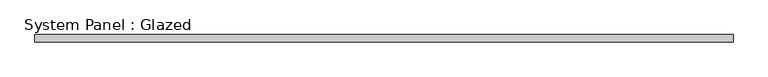
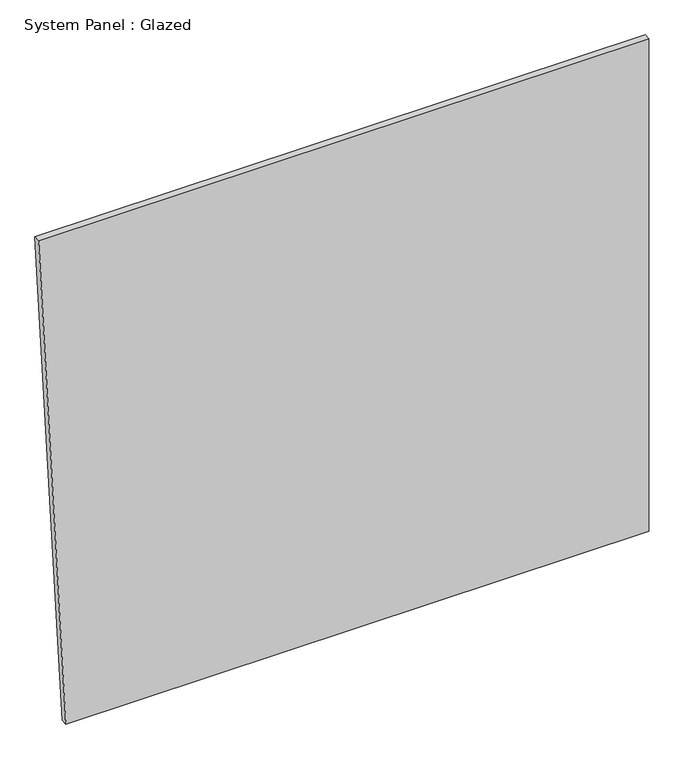
"""IFC4 building model written with IfcOpenShell, lengths in millimetres: plate geometry, System Panel : Glazed."""

import ifcopenshell
import ifcopenshell.guid

model = None  # the IFC model being written
_history = None  # IfcOwnerHistory: only IFC2X3 demands one
_inside = {}  # id of a spatial element -> (the spatial element, [elements in it])
_under = {}  # id of a project, library or spatial element -> (it, [spatial elements below it])
_declared = {}  # id of a project -> (the project, [libraries it declares])
_typed = {}  # id of a type object -> (the type object, [elements of that type])
_made_of = {}  # id of a material, layer set ... -> (it, [elements and type objects made of it])


def new_model(schema):
    """Start an empty IFC model of exactly this schema.

    Asked for "IFC4X3", IfcOpenShell would pick the latest addendum, in which some entities
    have other attributes; the version numbers below select the first issue.
    IFC2X3 requires an IfcOwnerHistory on every rooted entity: one is made here for all.
    """
    global model, _history
    if schema == "IFC4X3":
        model = ifcopenshell.file(schema_version=(4, 3, 0, 0))
    else:
        model = ifcopenshell.file(schema=schema)
    _inside.clear()
    _under.clear()
    _declared.clear()
    _typed.clear()
    _made_of.clear()
    _history = None
    if model.schema == "IFC2X3":
        org = make("IfcOrganization", Name="unknown")
        user = make(
            "IfcPersonAndOrganization",
            ThePerson=make("IfcPerson", FamilyName="unknown"),
            TheOrganization=org,
        )
        app = make(
            "IfcApplication",
            ApplicationDeveloper=org,
            Version="unknown",
            ApplicationFullName="unknown",
            ApplicationIdentifier="unknown",
        )
        _history = make(
            "IfcOwnerHistory",
            OwningUser=user,
            OwningApplication=app,
            ChangeAction="ADDED",
            CreationDate=0,
        )
    return model


def make(cls, **values):
    """One entity of the class cls with the attributes given. An attribute that is None is left unset."""
    return model.create_entity(
        cls, **{name: value for name, value in values.items() if value is not None}
    )


def rooted(cls, **values):
    """An entity with a GlobalId (a new one), such as an element, a storey or a relation."""
    return make(cls, GlobalId=ifcopenshell.guid.new(), OwnerHistory=_history, **values)


def si_unit(unit_type, name, prefix=None):
    """IfcSIUnit, for example si_unit("LENGTHUNIT", "METRE", prefix="MILLI")."""
    return make("IfcSIUnit", UnitType=unit_type, Prefix=prefix, Name=name)


def assignment(units):
    """IfcUnitAssignment: the units of a project."""
    return None if units is None else make("IfcUnitAssignment", Units=units)


def point(xyz):
    """IfcCartesianPoint."""
    return None if xyz is None else make("IfcCartesianPoint", Coordinates=xyz)


def direction(xyz):
    """IfcDirection."""
    return None if xyz is None else make("IfcDirection", DirectionRatios=xyz)


def frame(location, z_axis=None, x_axis=None):
    """IfcAxis2Placement3D, a coordinate frame: its origin and axes. An axis left out is left unset."""
    return make(
        "IfcAxis2Placement3D",
        Location=point(location),
        Axis=direction(z_axis),
        RefDirection=direction(x_axis),
    )


def origin():
    """The frame at (0, 0, 0) with its axes left unset."""
    return frame((0.0, 0.0, 0.0))


def place(relative_to, where):
    """IfcLocalPlacement: puts the frame where relative to a parent placement (None: the world)."""
    return make(
        "IfcLocalPlacement", PlacementRelTo=relative_to, RelativePlacement=where
    )


def context(
    kind, dimensions, precision=None, world=None, true_north=None, identifier=None
):
    """IfcGeometricRepresentationContext, for example the 3D "Model" context."""
    return make(
        "IfcGeometricRepresentationContext",
        ContextIdentifier=identifier,
        ContextType=kind,
        CoordinateSpaceDimension=dimensions,
        Precision=precision,
        WorldCoordinateSystem=world,
        TrueNorth=true_north,
    )


def project(units=None, contexts=None):
    """IfcProject with its units and contexts."""
    return rooted(
        "IfcProject",
        Name="project",
        RepresentationContexts=contexts,
        UnitsInContext=assignment(units),
    )


def spatial(cls, under=None, at=None, **own):
    """A site, building, storey or space (cls), placed at a placement, below another one or the project."""
    s = rooted(cls, ObjectPlacement=at, **own)
    if under is not None:
        _under.setdefault(under.id(), (under, []))[1].append(s)
    return s


def polyline(points):
    """IfcPolyline through the points."""
    return make("IfcPolyline", Points=[point(p) for p in points])


def outline(outer, holes=None, kind="AREA"):
    """IfcArbitraryClosedProfileDef: a profile drawn as a closed curve; with holes, ...WithVoids."""
    if holes is None:
        return make("IfcArbitraryClosedProfileDef", ProfileType=kind, OuterCurve=outer)
    return make(
        "IfcArbitraryProfileDefWithVoids",
        ProfileType=kind,
        OuterCurve=outer,
        InnerCurves=holes,
    )


def extrude(swept, where, along, depth):
    """IfcExtrudedAreaSolid: the profile swept, set in the frame where, extruded along a direction by depth."""
    return make(
        "IfcExtrudedAreaSolid",
        SweptArea=swept,
        Position=where,
        ExtrudedDirection=direction(along),
        Depth=depth,
    )


def shape(context_of_items, identifier, shape_type, items):
    """IfcShapeRepresentation: the items that make up one representation, for example the "Body"."""
    return make(
        "IfcShapeRepresentation",
        ContextOfItems=context_of_items,
        RepresentationIdentifier=identifier,
        RepresentationType=shape_type,
        Items=items,
    )


def source(mapping_origin, context_of_items, identifier, shape_type, items):
    """IfcRepresentationMap: a shape defined once, which mapped items show again and again."""
    return make(
        "IfcRepresentationMap",
        MappingOrigin=mapping_origin,
        MappedRepresentation=shape(context_of_items, identifier, shape_type, items),
    )


def transform(
    local_origin,
    x_axis=None,
    y_axis=None,
    z_axis=None,
    scale=None,
    scale2=None,
    scale3=None,
    uniform=True,
):
    """IfcCartesianTransformationOperator3D, or its non-uniform kind. x_axis, y_axis, z_axis: its Axis1, 2, 3."""
    if uniform:
        return make(
            "IfcCartesianTransformationOperator3D",
            Axis1=direction(x_axis),
            Axis2=direction(y_axis),
            LocalOrigin=point(local_origin),
            Scale=scale,
            Axis3=direction(z_axis),
        )
    return make(
        "IfcCartesianTransformationOperator3DnonUniform",
        Axis1=direction(x_axis),
        Axis2=direction(y_axis),
        LocalOrigin=point(local_origin),
        Scale=scale,
        Axis3=direction(z_axis),
        Scale2=scale2,
        Scale3=scale3,
    )


def mapped(mapping_source, mapping_target):
    """IfcMappedItem: shows the shape of a source again, moved by a transform."""
    return make(
        "IfcMappedItem", MappingSource=mapping_source, MappingTarget=mapping_target
    )


def made_of(thing, what):
    """Note that an element or type object is made of a material, layer set ...; save() writes the relation."""
    if what is not None:
        _made_of.setdefault(what.id(), (what, []))[1].append(thing)
    return thing


def element(
    cls,
    number,
    at=None,
    inside=None,
    cuts=None,
    type_object=None,
    material=None,
    context=None,
    identifier="Body",
    shape_type=None,
    held_by="IfcProductDefinitionShape",
    body=None,
    shapes=None,
    **own,
):
    """One element of the class cls, such as IfcWall. Its Tag is "e" and its number.

    at: its placement. inside: the storey or other place that contains it. cuts: it is an
    opening in that element (IfcRelVoidsElement). A single representation is given by context,
    identifier, shape_type and body (its items); several are given by shapes. held_by: the class
    of the entity that holds the representations. save() writes the other relations.
    """
    e = rooted(cls, Tag="e%d" % number, ObjectPlacement=at, **own)
    if body is not None:
        shapes = [shape(context, identifier, shape_type, body)]
    if shapes is not None:
        e.Representation = make(held_by, Representations=shapes)
    if inside is not None:
        _inside.setdefault(inside.id(), (inside, []))[1].append(e)
    if cuts is not None:
        rooted(
            "IfcRelVoidsElement", RelatingBuildingElement=cuts, RelatedOpeningElement=e
        )
    if type_object is not None:
        _typed.setdefault(type_object.id(), (type_object, []))[1].append(e)
    return made_of(e, material)


def aggregate(whole, parts):
    """IfcRelAggregates: a whole, such as a stair, and the parts it consists of."""
    return rooted("IfcRelAggregates", RelatingObject=whole, RelatedObjects=parts)


def save(model, path):
    """Write the relations noted so far, then the file.

    IfcRelAggregates (storeys below a building ...), IfcRelContainedInSpatialStructure (elements
    in a storey), IfcRelDefinesByType, IfcRelAssociatesMaterial and IfcRelDeclares: one each for
    every whole, place, type object, material and project.
    """
    for whole, parts in _under.values():
        aggregate(whole, parts)
    for where, things in _inside.values():
        rooted(
            "IfcRelContainedInSpatialStructure",
            RelatedElements=things,
            RelatingStructure=where,
        )
    for kind, things in _typed.values():
        rooted("IfcRelDefinesByType", RelatedObjects=things, RelatingType=kind)
    for what, things in _made_of.values():
        rooted("IfcRelAssociatesMaterial", RelatedObjects=things, RelatingMaterial=what)
    for by, libraries in _declared.values():
        rooted("IfcRelDeclares", RelatingContext=by, RelatedDefinitions=libraries)
    model.write(path)


def system_panel_glazed_bdf74c23(model_context):
    return source(origin(), model_context, "Body", "SweptSolid", [
        extrude(outline(polyline([(0.0, -1112.8894655), (0.0, 1222.0297486), (2085.3785982, 1222.0297486), (2085.3785982, -1222.0297486), (0.0, -1112.8894655)])), frame((0.0, -44.45, 0.0), z_axis=(0.0, 1.0, 0.0), x_axis=(0.0, 0.0, 1.0)), (0.0, 0.0, 1.0), 25.4),
    ])


if __name__ == "__main__":
    model = new_model("IFC4")
    model_context = context("Model", 3, world=origin())
    ifc_project = project(units=[si_unit("LENGTHUNIT", "METRE", prefix="MILLI")], contexts=[model_context])
    site = spatial("IfcSite", under=ifc_project)
    building = spatial("IfcBuilding", under=site)
    placement = place(None, origin())
    system_panel_glazed_shape = system_panel_glazed_bdf74c23(model_context)
    element("IfcPlate", 1, ObjectType="System Panel : Glazed", at=placement, inside=building, context=model_context, shape_type="MappedRepresentation", body=[
        mapped(system_panel_glazed_shape, transform((0.0, 0.0, 0.0), x_axis=(1.0, 0.0, 0.0), y_axis=(0.0, 1.0, 0.0), z_axis=(0.0, 0.0, 1.0))),
    ])
    save(model, "model.ifc")

# Revit data of these elements
# Type "System Panel : Glazed"
#   Construction Type Id = "GSP4R"
#   Analytic Construction = "1/8 in Pilkington single glazing"
#   Visual Light Transmittance = 0.9
#   Solar Heat Gain Coefficient = 0.86
#   Heat Transfer Coefficient (U) = 1.18115 BTU/(h·ft²·°F)
#   Define Thermal Properties by = 1
# Element 1 (IfcPlate, "System Panel : Glazed")
#   Materials on its faces: "Glass"
# Materials
#   "Glass": class "Glass", colour RGB 0 128 192, transparency 0.75, Description = "Soda Lime Glass", Cost = 0
